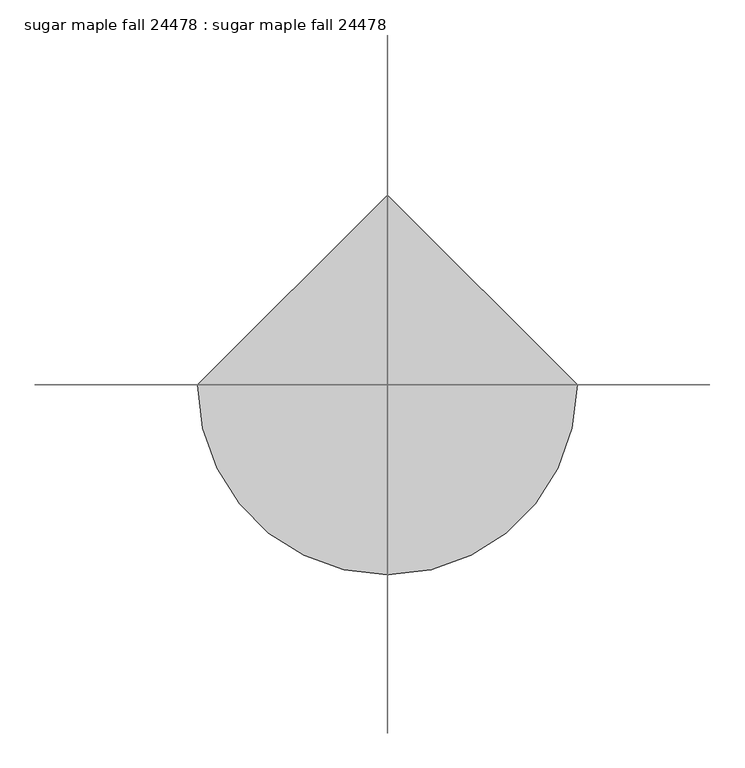
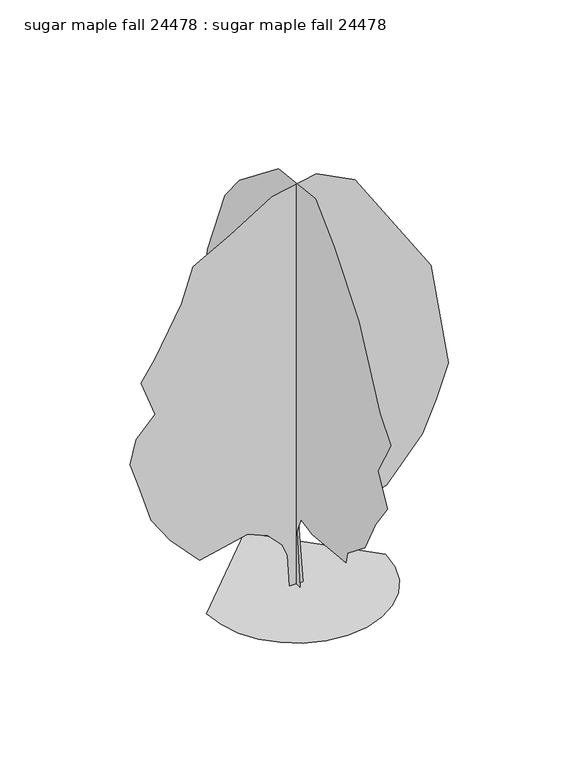
"""IFC4 building model written with IfcOpenShell, lengths in millimetres: proxy geometry, sugar maple fall 24478 : sugar maple fall 24478."""

from ifc_helpers import new_model, si_unit, origin, place, context, project, spatial, triangles, source, transform, mapped, element, save


def sugar_maple_fall_24478_sugar_maple_fall_24478_f594c2a4(model_context):
    return source(origin(), model_context, "Body", "Tessellation", [
        triangles([(-2874.6675568, 0.0, 9.75e-05), (-2798.670742, -658.6848673, 9.75e-05), (-2582.2377319, -1263.582756, 9.75e-05), (-2242.6907249, -1797.3631107, 9.75e-05), (-1797.3631107, -2242.6907249, 9.75e-05), (-1263.582756, -2582.2377319, 9.75e-05), (-658.6848673, -2798.670742, 9.75e-05), (0.0001257, -2874.6675568, 9.75e-05), (658.6848673, -2798.670742, 9.75e-05), (1263.582756, -2582.2377319, 9.75e-05), (1797.3631107, -2242.6907249, 9.75e-05), (2242.6907249, -1797.3631107, 9.75e-05), (2582.2377319, -1263.582756, 9.75e-05), (2798.670742, -658.6848673, 9.75e-05), (2874.6675568, 0.0002513, 9.75e-05), (-0.000377, 2874.6675568, 9.75e-05), (-2.08e-05, -199.1749247, 0.0346819), (4.82e-05, -56.8278721, 1817.6527153), (4.28e-05, -258.825735, 2341.1232342), (-2.85e-05, -903.7539202, 2207.885146), (-0.0001313, -1923.2734486, 2325.3143154), (-0.0002189, -2782.6179428, 2395.771352), (-0.0002163, -2865.4727692, 2771.5436188), (-0.0002948, -3839.4857002, 3546.573056), (-0.0003217, -4426.6312569, 4697.3949623), (-0.000363, -5084.2367569, 5613.3434143), (-0.0002773, -4544.0807739, 6599.7518097), (-0.0003147, -5272.145636, 7891.4671509), (-0.0002294, -4661.5050018, 8619.5320129), (-3.55e-05, -3487.2133072, 11015.1055573), (0.0001602, -2101.5355328, 12729.5788147), (0.0002973, -1068.1552952, 13715.9860474), (0.0005042, 975.1202763, 13504.608252), (0.0006798, 3149.1141769, 11787.0619263), (0.0007341, 3951.829715, 10801.5674286), (0.0007632, 4920.7624329, 8384.6841385), (0.0007481, 5085.151236, 7304.3215942), (0.0007261, 5296.5296127, 5824.7223724), (0.0005924, 4591.9598282, 3804.9162987), (0.0004639, 3629.0215118, 2865.4980583), (0.0004296, 3394.1733467, 2536.687896), (0.000374, 3092.6501816, 1726.1010361), (0.0002152, 1413.0031414, 2273.7472595), (0.0001457, 838.2271059, 1956.0621449), (7.66e-05, 382.876666, 1230.9488468), (2.05e-05, 196.9107642, 0.0347055), (-208.8982774, 9.1e-06, 0.0), (-283.5907205, -0.0001144, 1063.8550489), (-449.8182921, -0.0001567, 1479.347929), (-896.9010681, -0.0001936, 1952.9405331), (-1571.0977066, -0.0001973, 2231.3700497), (-3097.6792351, -8.98e-05, 1888.9910934), (-4045.0475716, -0.0001676, 2888.9678467), (-4666.6866623, -0.0002479, 3790.7939049), (-5023.5305786, -0.0003684, 4932.2431274), (-5340.7001724, -0.0004707, 5906.815036), (-5145.0190933, -0.0005731, 6693.7059586), (-4530.3141724, -0.0006783, 7351.3111679), (-4976.5660034, -0.0008016, 8549.0729416), (-4535.8766235, -0.0009022, 9231.2400238), (-3684.8250824, -0.0011268, 10803.7265991), (-3309.0579025, -0.0012773, 11928.3870209), (-2120.356913, -0.0014059, 12571.4384674), (-772.575808, -0.0015649, 13410.6791016), (660.0640709, -0.0016611, 13692.4909698), (1888.2468075, -0.0016387, 13054.2148132), (4323.8631111, -0.0012977, 9300.6322998), (4887.5394608, -0.0009052, 5801.2272949), (4511.746701, -0.0007572, 4697.3949623), (4053.9121468, -0.0006156, 3677.2051987), (2902.7853172, -0.0004043, 2327.2396339), (1552.5302353, -0.0003087, 2019.9964691), (433.9357224, -0.0003079, 2424.0719501), (75.5588282, -0.0002467, 2041.512743), (218.1486939, -9.5e-06, 0.0310248)], [[15, 16, 1], [14, 15, 1], [14, 1, 2], [13, 14, 2], [13, 2, 3], [13, 3, 4], [12, 13, 4], [11, 12, 4], [11, 4, 5], [11, 5, 6], [11, 6, 7], [11, 7, 8], [11, 8, 9], [11, 9, 10], [46, 17, 18], [45, 46, 18], [44, 45, 18], [41, 42, 43], [44, 18, 19], [21, 22, 23], [27, 28, 29], [25, 26, 27], [31, 32, 33], [31, 33, 34], [30, 31, 34], [30, 34, 35], [30, 35, 36], [29, 30, 36], [27, 29, 36], [27, 36, 37], [25, 27, 37], [24, 25, 37], [23, 24, 37], [21, 23, 37], [20, 21, 37], [19, 20, 37], [19, 37, 38], [19, 38, 39], [19, 39, 40], [19, 40, 41], [19, 41, 43], [44, 19, 43], [74, 75, 47], [74, 47, 48], [74, 48, 49], [74, 49, 50], [51, 52, 53], [58, 59, 60], [61, 62, 63], [73, 74, 50], [73, 50, 51], [51, 53, 54], [51, 54, 55], [73, 51, 55], [73, 55, 56], [73, 56, 57], [73, 57, 58], [73, 58, 60], [73, 60, 61], [73, 61, 63], [73, 63, 64], [73, 64, 65], [73, 65, 66], [73, 66, 67], [73, 67, 68], [73, 68, 69], [73, 69, 70], [73, 70, 71], [73, 71, 72]], closed=False),
    ])


if __name__ == "__main__":
    model = new_model("IFC4")
    model_context = context("Model", 3, world=origin())
    ifc_project = project(units=[si_unit("LENGTHUNIT", "METRE", prefix="MILLI")], contexts=[model_context])
    site = spatial("IfcSite", under=ifc_project)
    building = spatial("IfcBuilding", under=site)
    placement = place(None, origin())
    sugar_maple_fall_24478_sugar_maple_fall_24478_shape = sugar_maple_fall_24478_sugar_maple_fall_24478_f594c2a4(model_context)
    element("IfcBuildingElementProxy", 1, Name="sugar maple fall 24478 : sugar maple fall 24478", ObjectType="sugar maple fall 24478 : sugar maple fall 24478", at=placement, inside=building, context=model_context, shape_type="MappedRepresentation", body=[
        mapped(sugar_maple_fall_24478_sugar_maple_fall_24478_shape, transform((0.0, 0.0, 0.0), x_axis=(1.0, 0.0, 0.0), y_axis=(0.0, 1.0, 0.0), z_axis=(0.0, 0.0, 1.0))),
    ])
    save(model, "model.ifc")

# Revit data of these elements
# Type "sugar maple fall 24478 : sugar maple fall 24478"
#   built-in parameter 1005195 = "RPC-16-FWM4-JJQ0-CAW1-2000-ST1L-LVER-AU"
#   Height = 0
